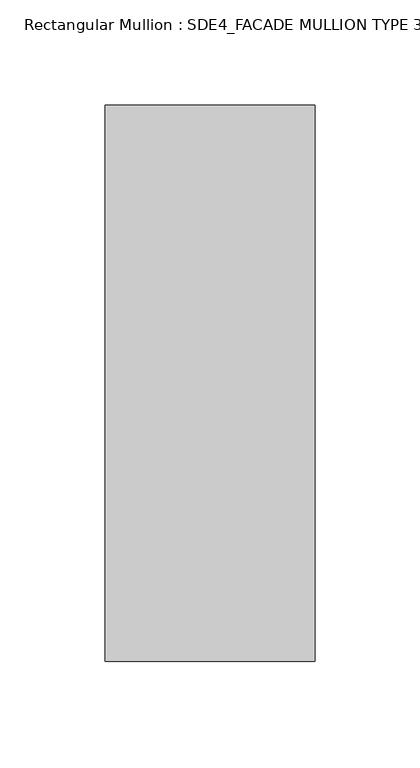
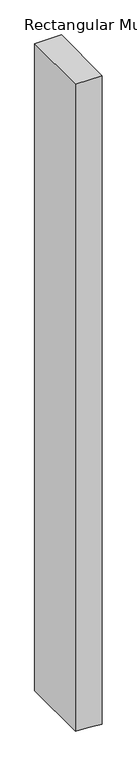
"""IFC4 building model written with IfcOpenShell, lengths in millimetres: member geometry, Rectangular Mullion : SDE4_FACADE MULLION TYPE 3."""

from ifc_helpers import new_model, si_unit, frame, origin, place, context, project, spatial, polyline, outline, extrude, source, transform, mapped, element, save


def rectangular_mullion_sde4_facade_mullion_type_3_bd9e27e1(model_context):
    return source(origin(), model_context, "Body", "SweptSolid", [
        extrude(outline(polyline([(0.0, 50.0), (0.0, -50.0), (-2560.261432, -50.0), (-2564.3275111, 3.056508), (-2567.9251084, 50.0), (0.0, 50.0)])), frame((0.0, -132.5, 0.0), z_axis=(0.0, 1.0, 0.0), x_axis=(0.0, 0.0, 1.0)), (0.0, 0.0, 1.0), 265.0),
    ])


if __name__ == "__main__":
    model = new_model("IFC4")
    model_context = context("Model", 3, world=origin())
    ifc_project = project(units=[si_unit("LENGTHUNIT", "METRE", prefix="MILLI")], contexts=[model_context])
    site = spatial("IfcSite", under=ifc_project)
    building = spatial("IfcBuilding", under=site)
    placement = place(None, origin())
    rectangular_mullion_sde4_facade_mullion_type_3_shape = rectangular_mullion_sde4_facade_mullion_type_3_bd9e27e1(model_context)
    element("IfcMember", 1, ObjectType="Rectangular Mullion : SDE4_FACADE MULLION TYPE 3", at=placement, inside=building, context=model_context, shape_type="MappedRepresentation", body=[
        mapped(rectangular_mullion_sde4_facade_mullion_type_3_shape, transform((0.0, 0.0, 0.0), x_axis=(1.0, 0.0, 0.0), y_axis=(0.0, 1.0, 0.0), z_axis=(0.0, 0.0, 1.0))),
    ])
    save(model, "model.ifc")

# Revit data of these elements
# Type "Rectangular Mullion : SDE4_FACADE MULLION TYPE 3"
#   built-in parameter 1007322 = 0.869423 (stored number, unit not read)
#   built-in parameter 1007321 = 0.164042 (stored number, unit not read)
#   built-in parameter 1007320 = 0.164042 (stored number, unit not read)
